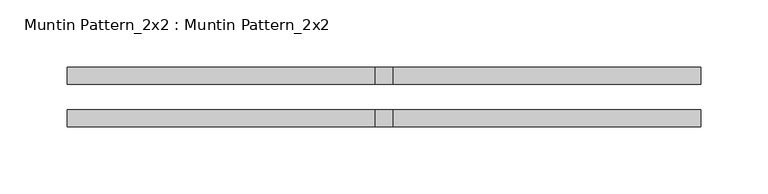
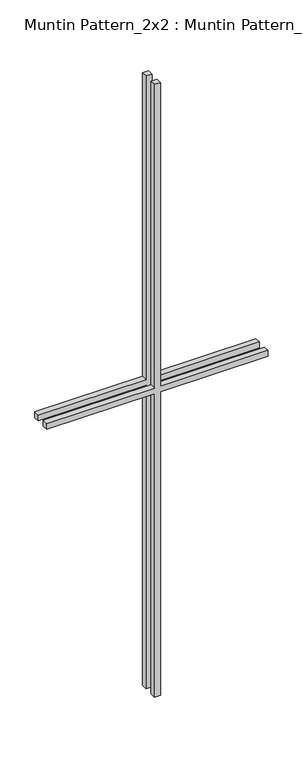
"""IFC4 building model written with IfcOpenShell, lengths in millimetres: proxy geometry, Muntin Pattern_2x2 : Muntin Pattern_2x2."""

import ifcopenshell
import ifcopenshell.guid

model = None  # the IFC model being written
_history = None  # IfcOwnerHistory: only IFC2X3 demands one
_inside = {}  # id of a spatial element -> (the spatial element, [elements in it])
_under = {}  # id of a project, library or spatial element -> (it, [spatial elements below it])
_declared = {}  # id of a project -> (the project, [libraries it declares])
_typed = {}  # id of a type object -> (the type object, [elements of that type])
_made_of = {}  # id of a material, layer set ... -> (it, [elements and type objects made of it])


def new_model(schema):
    """Start an empty IFC model of exactly this schema.

    Asked for "IFC4X3", IfcOpenShell would pick the latest addendum, in which some entities
    have other attributes; the version numbers below select the first issue.
    IFC2X3 requires an IfcOwnerHistory on every rooted entity: one is made here for all.
    """
    global model, _history
    if schema == "IFC4X3":
        model = ifcopenshell.file(schema_version=(4, 3, 0, 0))
    else:
        model = ifcopenshell.file(schema=schema)
    _inside.clear()
    _under.clear()
    _declared.clear()
    _typed.clear()
    _made_of.clear()
    _history = None
    if model.schema == "IFC2X3":
        org = make("IfcOrganization", Name="unknown")
        user = make(
            "IfcPersonAndOrganization",
            ThePerson=make("IfcPerson", FamilyName="unknown"),
            TheOrganization=org,
        )
        app = make(
            "IfcApplication",
            ApplicationDeveloper=org,
            Version="unknown",
            ApplicationFullName="unknown",
            ApplicationIdentifier="unknown",
        )
        _history = make(
            "IfcOwnerHistory",
            OwningUser=user,
            OwningApplication=app,
            ChangeAction="ADDED",
            CreationDate=0,
        )
    return model


def make(cls, **values):
    """One entity of the class cls with the attributes given. An attribute that is None is left unset."""
    return model.create_entity(
        cls, **{name: value for name, value in values.items() if value is not None}
    )


def rooted(cls, **values):
    """An entity with a GlobalId (a new one), such as an element, a storey or a relation."""
    return make(cls, GlobalId=ifcopenshell.guid.new(), OwnerHistory=_history, **values)


def si_unit(unit_type, name, prefix=None):
    """IfcSIUnit, for example si_unit("LENGTHUNIT", "METRE", prefix="MILLI")."""
    return make("IfcSIUnit", UnitType=unit_type, Prefix=prefix, Name=name)


def assignment(units):
    """IfcUnitAssignment: the units of a project."""
    return None if units is None else make("IfcUnitAssignment", Units=units)


def point(xyz):
    """IfcCartesianPoint."""
    return None if xyz is None else make("IfcCartesianPoint", Coordinates=xyz)


def direction(xyz):
    """IfcDirection."""
    return None if xyz is None else make("IfcDirection", DirectionRatios=xyz)


def frame(location, z_axis=None, x_axis=None):
    """IfcAxis2Placement3D, a coordinate frame: its origin and axes. An axis left out is left unset."""
    return make(
        "IfcAxis2Placement3D",
        Location=point(location),
        Axis=direction(z_axis),
        RefDirection=direction(x_axis),
    )


def origin():
    """The frame at (0, 0, 0) with its axes left unset."""
    return frame((0.0, 0.0, 0.0))


def place(relative_to, where):
    """IfcLocalPlacement: puts the frame where relative to a parent placement (None: the world)."""
    return make(
        "IfcLocalPlacement", PlacementRelTo=relative_to, RelativePlacement=where
    )


def context(
    kind, dimensions, precision=None, world=None, true_north=None, identifier=None
):
    """IfcGeometricRepresentationContext, for example the 3D "Model" context."""
    return make(
        "IfcGeometricRepresentationContext",
        ContextIdentifier=identifier,
        ContextType=kind,
        CoordinateSpaceDimension=dimensions,
        Precision=precision,
        WorldCoordinateSystem=world,
        TrueNorth=true_north,
    )


def project(units=None, contexts=None):
    """IfcProject with its units and contexts."""
    return rooted(
        "IfcProject",
        Name="project",
        RepresentationContexts=contexts,
        UnitsInContext=assignment(units),
    )


def spatial(cls, under=None, at=None, **own):
    """A site, building, storey or space (cls), placed at a placement, below another one or the project."""
    s = rooted(cls, ObjectPlacement=at, **own)
    if under is not None:
        _under.setdefault(under.id(), (under, []))[1].append(s)
    return s


def polyline(points):
    """IfcPolyline through the points."""
    return make("IfcPolyline", Points=[point(p) for p in points])


def outline(outer, holes=None, kind="AREA"):
    """IfcArbitraryClosedProfileDef: a profile drawn as a closed curve; with holes, ...WithVoids."""
    if holes is None:
        return make("IfcArbitraryClosedProfileDef", ProfileType=kind, OuterCurve=outer)
    return make(
        "IfcArbitraryProfileDefWithVoids",
        ProfileType=kind,
        OuterCurve=outer,
        InnerCurves=holes,
    )


def extrude(swept, where, along, depth):
    """IfcExtrudedAreaSolid: the profile swept, set in the frame where, extruded along a direction by depth."""
    return make(
        "IfcExtrudedAreaSolid",
        SweptArea=swept,
        Position=where,
        ExtrudedDirection=direction(along),
        Depth=depth,
    )


def shape(context_of_items, identifier, shape_type, items):
    """IfcShapeRepresentation: the items that make up one representation, for example the "Body"."""
    return make(
        "IfcShapeRepresentation",
        ContextOfItems=context_of_items,
        RepresentationIdentifier=identifier,
        RepresentationType=shape_type,
        Items=items,
    )


def source(mapping_origin, context_of_items, identifier, shape_type, items):
    """IfcRepresentationMap: a shape defined once, which mapped items show again and again."""
    return make(
        "IfcRepresentationMap",
        MappingOrigin=mapping_origin,
        MappedRepresentation=shape(context_of_items, identifier, shape_type, items),
    )


def transform(
    local_origin,
    x_axis=None,
    y_axis=None,
    z_axis=None,
    scale=None,
    scale2=None,
    scale3=None,
    uniform=True,
):
    """IfcCartesianTransformationOperator3D, or its non-uniform kind. x_axis, y_axis, z_axis: its Axis1, 2, 3."""
    if uniform:
        return make(
            "IfcCartesianTransformationOperator3D",
            Axis1=direction(x_axis),
            Axis2=direction(y_axis),
            LocalOrigin=point(local_origin),
            Scale=scale,
            Axis3=direction(z_axis),
        )
    return make(
        "IfcCartesianTransformationOperator3DnonUniform",
        Axis1=direction(x_axis),
        Axis2=direction(y_axis),
        LocalOrigin=point(local_origin),
        Scale=scale,
        Axis3=direction(z_axis),
        Scale2=scale2,
        Scale3=scale3,
    )


def mapped(mapping_source, mapping_target):
    """IfcMappedItem: shows the shape of a source again, moved by a transform."""
    return make(
        "IfcMappedItem", MappingSource=mapping_source, MappingTarget=mapping_target
    )


def made_of(thing, what):
    """Note that an element or type object is made of a material, layer set ...; save() writes the relation."""
    if what is not None:
        _made_of.setdefault(what.id(), (what, []))[1].append(thing)
    return thing


def element(
    cls,
    number,
    at=None,
    inside=None,
    cuts=None,
    type_object=None,
    material=None,
    context=None,
    identifier="Body",
    shape_type=None,
    held_by="IfcProductDefinitionShape",
    body=None,
    shapes=None,
    **own,
):
    """One element of the class cls, such as IfcWall. Its Tag is "e" and its number.

    at: its placement. inside: the storey or other place that contains it. cuts: it is an
    opening in that element (IfcRelVoidsElement). A single representation is given by context,
    identifier, shape_type and body (its items); several are given by shapes. held_by: the class
    of the entity that holds the representations. save() writes the other relations.
    """
    e = rooted(cls, Tag="e%d" % number, ObjectPlacement=at, **own)
    if body is not None:
        shapes = [shape(context, identifier, shape_type, body)]
    if shapes is not None:
        e.Representation = make(held_by, Representations=shapes)
    if inside is not None:
        _inside.setdefault(inside.id(), (inside, []))[1].append(e)
    if cuts is not None:
        rooted(
            "IfcRelVoidsElement", RelatingBuildingElement=cuts, RelatedOpeningElement=e
        )
    if type_object is not None:
        _typed.setdefault(type_object.id(), (type_object, []))[1].append(e)
    return made_of(e, material)


def aggregate(whole, parts):
    """IfcRelAggregates: a whole, such as a stair, and the parts it consists of."""
    return rooted("IfcRelAggregates", RelatingObject=whole, RelatedObjects=parts)


def save(model, path):
    """Write the relations noted so far, then the file.

    IfcRelAggregates (storeys below a building ...), IfcRelContainedInSpatialStructure (elements
    in a storey), IfcRelDefinesByType, IfcRelAssociatesMaterial and IfcRelDeclares: one each for
    every whole, place, type object, material and project.
    """
    for whole, parts in _under.values():
        aggregate(whole, parts)
    for where, things in _inside.values():
        rooted(
            "IfcRelContainedInSpatialStructure",
            RelatedElements=things,
            RelatingStructure=where,
        )
    for kind, things in _typed.values():
        rooted("IfcRelDefinesByType", RelatedObjects=things, RelatingType=kind)
    for what, things in _made_of.values():
        rooted("IfcRelAssociatesMaterial", RelatedObjects=things, RelatingMaterial=what)
    for by, libraries in _declared.values():
        rooted("IfcRelDeclares", RelatingContext=by, RelatedDefinitions=libraries)
    model.write(path)


def muntin_pattern_2x2_muntin_pattern_2x2_6dad3731(model_context):
    return source(origin(), model_context, "Body", "SweptSolid", [
        extrude(outline(polyline([(698.5, -6.35), (698.5, -236.5375), (685.8, -236.5375), (685.8, -6.35), (0.0, -6.35), (0.0, 6.35), (685.8, 6.35), (685.8, 236.5375), (698.5, 236.5375), (698.5, 6.35), (1384.3, 6.35), (1384.3, -6.35), (698.5, -6.35)])), frame((0.0, 9.525, 0.0), z_axis=(0.0, 1.0, 0.0), x_axis=(0.0, 0.0, 1.0)), (0.0, 0.0, 1.0), 12.7),
        extrude(outline(polyline([(698.5, -6.35), (698.5, -236.5375), (685.8, -236.5375), (685.8, -6.35), (0.0, -6.35), (0.0, 6.35), (685.8, 6.35), (685.8, 236.5375), (698.5, 236.5375), (698.5, 6.35), (1384.3, 6.35), (1384.3, -6.35), (698.5, -6.35)])), frame((0.0, -22.225, 0.0), z_axis=(0.0, 1.0, 0.0), x_axis=(0.0, 0.0, 1.0)), (0.0, 0.0, 1.0), 12.7),
    ])


if __name__ == "__main__":
    model = new_model("IFC4")
    model_context = context("Model", 3, world=origin())
    ifc_project = project(units=[si_unit("LENGTHUNIT", "METRE", prefix="MILLI")], contexts=[model_context])
    site = spatial("IfcSite", under=ifc_project)
    building = spatial("IfcBuilding", under=site)
    placement = place(None, origin())
    muntin_pattern_2x2_muntin_pattern_2x2_shape = muntin_pattern_2x2_muntin_pattern_2x2_6dad3731(model_context)
    element("IfcBuildingElementProxy", 1, Name="Muntin Pattern_2x2 : Muntin Pattern_2x2", ObjectType="Muntin Pattern_2x2 : Muntin Pattern_2x2", at=placement, inside=building, context=model_context, shape_type="MappedRepresentation", body=[
        mapped(muntin_pattern_2x2_muntin_pattern_2x2_shape, transform((0.0, 0.0, 0.0), x_axis=(1.0, 0.0, 0.0), y_axis=(0.0, 1.0, 0.0), z_axis=(0.0, 0.0, 1.0))),
    ])
    save(model, "model.ifc")

# Revit data of these elements
# Type "Muntin Pattern_2x2 : Muntin Pattern_2x2"
#   Width [instance default] = 4' - 0"
#   Thickness = 0' - 0 1/2"
#   Height [instance default] = 4' - 0"
#   Distance = 0' - 0 3/4"
#   Interior Material [instance default] = none
#   Exterior Material [instance default] = none
#   Default Elevation = 0
# Element 1 (IfcBuildingElementProxy, "Muntin Pattern_2x2 : Muntin Pattern_2x2")
#   Width = 1' - 6 5/8"
#   Height = 4' - 6 1/2"
#   Interior Material = Wood - Stained
#   Exterior Material = Clad - White
#   Materials on its faces: "Clad - White", "Wood - Stained"
# Materials
#   "Clad - White": class "Wood", colour RGB 216 216 204, transparency 0, Cost = 0
#   "Wood - Stained": class "Wood", colour RGB 224 178 126, transparency 0, Cost = 0
